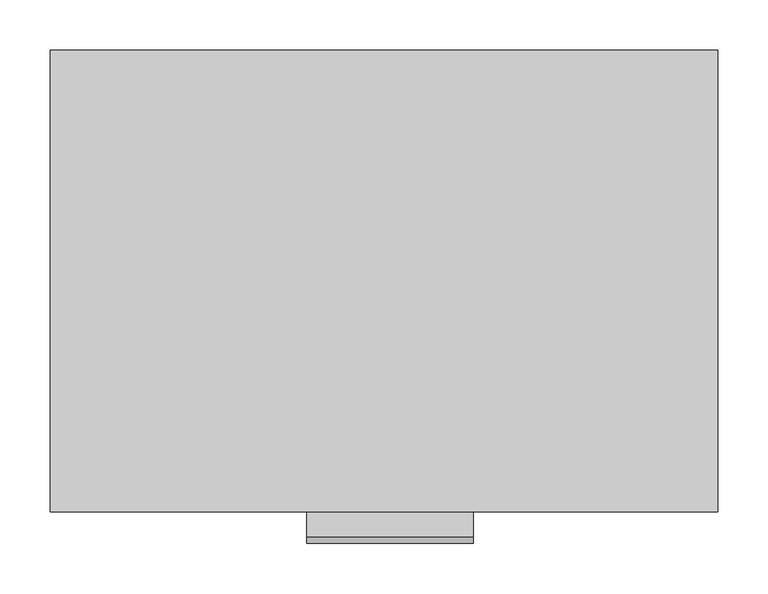
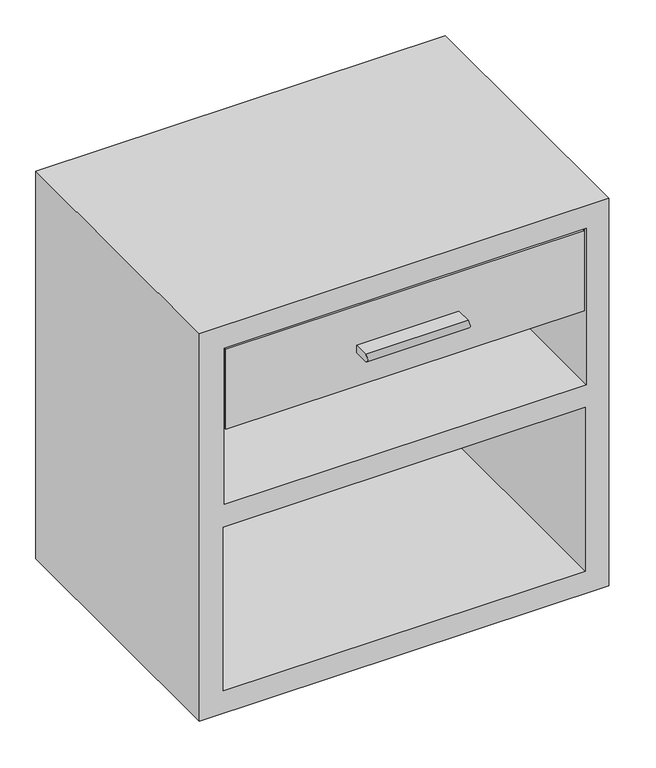
"""IFC4 building model written with IfcOpenShell, lengths in millimetres: furniture geometry, Livia_1_Drawer_Nightstand_20913 : Livia_1_Drawer_Nightstand_20913."""

import ifcopenshell
import ifcopenshell.guid

model = None  # the IFC model being written
_history = None  # IfcOwnerHistory: only IFC2X3 demands one
_inside = {}  # id of a spatial element -> (the spatial element, [elements in it])
_under = {}  # id of a project, library or spatial element -> (it, [spatial elements below it])
_declared = {}  # id of a project -> (the project, [libraries it declares])
_typed = {}  # id of a type object -> (the type object, [elements of that type])
_made_of = {}  # id of a material, layer set ... -> (it, [elements and type objects made of it])


def new_model(schema):
    """Start an empty IFC model of exactly this schema.

    Asked for "IFC4X3", IfcOpenShell would pick the latest addendum, in which some entities
    have other attributes; the version numbers below select the first issue.
    IFC2X3 requires an IfcOwnerHistory on every rooted entity: one is made here for all.
    """
    global model, _history
    if schema == "IFC4X3":
        model = ifcopenshell.file(schema_version=(4, 3, 0, 0))
    else:
        model = ifcopenshell.file(schema=schema)
    _inside.clear()
    _under.clear()
    _declared.clear()
    _typed.clear()
    _made_of.clear()
    _history = None
    if model.schema == "IFC2X3":
        org = make("IfcOrganization", Name="unknown")
        user = make(
            "IfcPersonAndOrganization",
            ThePerson=make("IfcPerson", FamilyName="unknown"),
            TheOrganization=org,
        )
        app = make(
            "IfcApplication",
            ApplicationDeveloper=org,
            Version="unknown",
            ApplicationFullName="unknown",
            ApplicationIdentifier="unknown",
        )
        _history = make(
            "IfcOwnerHistory",
            OwningUser=user,
            OwningApplication=app,
            ChangeAction="ADDED",
            CreationDate=0,
        )
    return model


def make(cls, **values):
    """One entity of the class cls with the attributes given. An attribute that is None is left unset."""
    return model.create_entity(
        cls, **{name: value for name, value in values.items() if value is not None}
    )


def rooted(cls, **values):
    """An entity with a GlobalId (a new one), such as an element, a storey or a relation."""
    return make(cls, GlobalId=ifcopenshell.guid.new(), OwnerHistory=_history, **values)


def si_unit(unit_type, name, prefix=None):
    """IfcSIUnit, for example si_unit("LENGTHUNIT", "METRE", prefix="MILLI")."""
    return make("IfcSIUnit", UnitType=unit_type, Prefix=prefix, Name=name)


def assignment(units):
    """IfcUnitAssignment: the units of a project."""
    return None if units is None else make("IfcUnitAssignment", Units=units)


def point(xyz):
    """IfcCartesianPoint."""
    return None if xyz is None else make("IfcCartesianPoint", Coordinates=xyz)


def direction(xyz):
    """IfcDirection."""
    return None if xyz is None else make("IfcDirection", DirectionRatios=xyz)


def frame(location, z_axis=None, x_axis=None):
    """IfcAxis2Placement3D, a coordinate frame: its origin and axes. An axis left out is left unset."""
    return make(
        "IfcAxis2Placement3D",
        Location=point(location),
        Axis=direction(z_axis),
        RefDirection=direction(x_axis),
    )


def origin():
    """The frame at (0, 0, 0) with its axes left unset."""
    return frame((0.0, 0.0, 0.0))


def place(relative_to, where):
    """IfcLocalPlacement: puts the frame where relative to a parent placement (None: the world)."""
    return make(
        "IfcLocalPlacement", PlacementRelTo=relative_to, RelativePlacement=where
    )


def context(
    kind, dimensions, precision=None, world=None, true_north=None, identifier=None
):
    """IfcGeometricRepresentationContext, for example the 3D "Model" context."""
    return make(
        "IfcGeometricRepresentationContext",
        ContextIdentifier=identifier,
        ContextType=kind,
        CoordinateSpaceDimension=dimensions,
        Precision=precision,
        WorldCoordinateSystem=world,
        TrueNorth=true_north,
    )


def project(units=None, contexts=None):
    """IfcProject with its units and contexts."""
    return rooted(
        "IfcProject",
        Name="project",
        RepresentationContexts=contexts,
        UnitsInContext=assignment(units),
    )


def spatial(cls, under=None, at=None, **own):
    """A site, building, storey or space (cls), placed at a placement, below another one or the project."""
    s = rooted(cls, ObjectPlacement=at, **own)
    if under is not None:
        _under.setdefault(under.id(), (under, []))[1].append(s)
    return s


def faces_of(points, faces, orient=None, outer=None):
    """IfcFace entities. A face is a list of loops; a loop is a list of indices into points, from 0.

    orient and outer hold one flag for each loop. By default every Orientation is true, the
    first loop of a face is its IfcFaceOuterBound and the others are IfcFaceBound.
    """
    made = []
    for i, loops in enumerate(faces):
        bounds = []
        for j, loop in enumerate(loops):
            is_outer = j == 0 if outer is None else outer[i][j]
            bounds.append(
                make(
                    "IfcFaceOuterBound" if is_outer else "IfcFaceBound",
                    Bound=make("IfcPolyLoop", Polygon=[points[k] for k in loop]),
                    Orientation=True if orient is None else orient[i][j],
                )
            )
        made.append(make("IfcFace", Bounds=bounds))
    return made


def faceted_brep(points, faces, orient=None, outer=None, voids=None):
    """IfcFacetedBrep: a solid bounded by flat faces; with voids (closed shells), ...WithVoids."""
    shared = [point(p) for p in points]
    hull = make("IfcClosedShell", CfsFaces=faces_of(shared, faces, orient, outer))
    if voids is None:
        return make("IfcFacetedBrep", Outer=hull)
    return make(
        "IfcFacetedBrepWithVoids",
        Outer=hull,
        Voids=[
            make(cls, CfsFaces=faces_of(shared, fs, o, b)) for cls, fs, o, b in voids
        ],
    )


def shape(context_of_items, identifier, shape_type, items):
    """IfcShapeRepresentation: the items that make up one representation, for example the "Body"."""
    return make(
        "IfcShapeRepresentation",
        ContextOfItems=context_of_items,
        RepresentationIdentifier=identifier,
        RepresentationType=shape_type,
        Items=items,
    )


def source(mapping_origin, context_of_items, identifier, shape_type, items):
    """IfcRepresentationMap: a shape defined once, which mapped items show again and again."""
    return make(
        "IfcRepresentationMap",
        MappingOrigin=mapping_origin,
        MappedRepresentation=shape(context_of_items, identifier, shape_type, items),
    )


def transform(
    local_origin,
    x_axis=None,
    y_axis=None,
    z_axis=None,
    scale=None,
    scale2=None,
    scale3=None,
    uniform=True,
):
    """IfcCartesianTransformationOperator3D, or its non-uniform kind. x_axis, y_axis, z_axis: its Axis1, 2, 3."""
    if uniform:
        return make(
            "IfcCartesianTransformationOperator3D",
            Axis1=direction(x_axis),
            Axis2=direction(y_axis),
            LocalOrigin=point(local_origin),
            Scale=scale,
            Axis3=direction(z_axis),
        )
    return make(
        "IfcCartesianTransformationOperator3DnonUniform",
        Axis1=direction(x_axis),
        Axis2=direction(y_axis),
        LocalOrigin=point(local_origin),
        Scale=scale,
        Axis3=direction(z_axis),
        Scale2=scale2,
        Scale3=scale3,
    )


def mapped(mapping_source, mapping_target):
    """IfcMappedItem: shows the shape of a source again, moved by a transform."""
    return make(
        "IfcMappedItem", MappingSource=mapping_source, MappingTarget=mapping_target
    )


def made_of(thing, what):
    """Note that an element or type object is made of a material, layer set ...; save() writes the relation."""
    if what is not None:
        _made_of.setdefault(what.id(), (what, []))[1].append(thing)
    return thing


def element(
    cls,
    number,
    at=None,
    inside=None,
    cuts=None,
    type_object=None,
    material=None,
    context=None,
    identifier="Body",
    shape_type=None,
    held_by="IfcProductDefinitionShape",
    body=None,
    shapes=None,
    **own,
):
    """One element of the class cls, such as IfcWall. Its Tag is "e" and its number.

    at: its placement. inside: the storey or other place that contains it. cuts: it is an
    opening in that element (IfcRelVoidsElement). A single representation is given by context,
    identifier, shape_type and body (its items); several are given by shapes. held_by: the class
    of the entity that holds the representations. save() writes the other relations.
    """
    e = rooted(cls, Tag="e%d" % number, ObjectPlacement=at, **own)
    if body is not None:
        shapes = [shape(context, identifier, shape_type, body)]
    if shapes is not None:
        e.Representation = make(held_by, Representations=shapes)
    if inside is not None:
        _inside.setdefault(inside.id(), (inside, []))[1].append(e)
    if cuts is not None:
        rooted(
            "IfcRelVoidsElement", RelatingBuildingElement=cuts, RelatedOpeningElement=e
        )
    if type_object is not None:
        _typed.setdefault(type_object.id(), (type_object, []))[1].append(e)
    return made_of(e, material)


def aggregate(whole, parts):
    """IfcRelAggregates: a whole, such as a stair, and the parts it consists of."""
    return rooted("IfcRelAggregates", RelatingObject=whole, RelatedObjects=parts)


def save(model, path):
    """Write the relations noted so far, then the file.

    IfcRelAggregates (storeys below a building ...), IfcRelContainedInSpatialStructure (elements
    in a storey), IfcRelDefinesByType, IfcRelAssociatesMaterial and IfcRelDeclares: one each for
    every whole, place, type object, material and project.
    """
    for whole, parts in _under.values():
        aggregate(whole, parts)
    for where, things in _inside.values():
        rooted(
            "IfcRelContainedInSpatialStructure",
            RelatedElements=things,
            RelatingStructure=where,
        )
    for kind, things in _typed.values():
        rooted("IfcRelDefinesByType", RelatedObjects=things, RelatingType=kind)
    for what, things in _made_of.values():
        rooted("IfcRelAssociatesMaterial", RelatedObjects=things, RelatingMaterial=what)
    for by, libraries in _declared.values():
        rooted("IfcRelDeclares", RelatingContext=by, RelatedDefinitions=libraries)
    model.write(path)


def plane_surface(at):
    """IfcPlane: the flat surface through the origin of the frame at, square to its z axis."""
    return make("IfcPlane", Position=at)


def extruded_surface(curve, direction_of_extrusion, depth):
    """IfcSurfaceOfLinearExtrusion: the curve pushed along a direction by depth."""
    return make(
        "IfcSurfaceOfLinearExtrusion",
        SweptCurve=make("IfcArbitraryOpenProfileDef", ProfileType="CURVE", Curve=curve),
        ExtrudedDirection=direction(direction_of_extrusion),
        Depth=depth,
    )


def spline_curve(degree, points, multiplicities, knots, weights=None):
    """IfcBSplineCurveWithKnots; with weights, IfcRationalBSplineCurveWithKnots."""
    own = dict(
        Degree=degree,
        ControlPointsList=[point(p) for p in points],
        CurveForm="UNSPECIFIED",
        ClosedCurve=False,
        SelfIntersect=False,
        KnotMultiplicities=multiplicities,
        Knots=knots,
        KnotSpec="UNSPECIFIED",
    )
    if weights is None:
        return make("IfcBSplineCurveWithKnots", **own)
    return make("IfcRationalBSplineCurveWithKnots", WeightsData=weights, **own)


def advanced_brep(points, edges, surfaces, faces):
    """IfcAdvancedBrep: a solid bounded by faces that lie on surfaces and meet in shared edges.

    An edge is (start, end): straight between two places in points (the first is 0);
    or (start, end, curve); or (start, end, curve, False) where it runs against its curve.
    A face is (place in surfaces, loops), or (place, loops, False) where it looks against
    its surface's normal. A loop lists edges by number (the first is 1), with a minus sign
    where the edge is run from its end to its start. The first loop is the outer one.
    """
    corners = [point(p) for p in points]
    vertices = [make("IfcVertexPoint", VertexGeometry=c) for c in corners]
    made = []
    for start, end, *more in edges:
        made.append(
            make(
                "IfcEdgeCurve",
                EdgeStart=vertices[start],
                EdgeEnd=vertices[end],
                EdgeGeometry=more[0] if more else make("IfcPolyline", Points=[corners[start], corners[end]]),
                SameSense=more[1] if len(more) > 1 else True,
            )
        )
    hull = []
    for where, loops, *sense in faces:
        bounds = []
        for j, loop in enumerate(loops):
            ring = [make("IfcOrientedEdge", EdgeElement=made[abs(k) - 1], Orientation=k > 0) for k in loop]
            bounds.append(
                make(
                    "IfcFaceOuterBound" if j == 0 else "IfcFaceBound",
                    Bound=make("IfcEdgeLoop", EdgeList=ring),
                    Orientation=True,
                )
            )
        hull.append(make("IfcAdvancedFace", Bounds=bounds, FaceSurface=surfaces[where], SameSense=sense[0] if sense else True))
    return make("IfcAdvancedBrep", Outer=make("IfcClosedShell", CfsFaces=hull))


def furniture_23f017af(model_context):
    return source(origin(), model_context, "Body", "SolidModel", [
        advanced_brep(
        [(-76.575761, -228.6, 552.45), (-76.575761, -228.6, 539.75), (-76.575761, -254.0, 539.75), (-76.575761, -254.0, 552.45), (88.524239, -228.6, 552.45), (88.524239, -254.0, 552.45), (88.524239, -254.0, 539.75), (88.524239, -228.6, 539.75)],
        [
            (0, 1),
            (1, 2),
            (2, 3, spline_curve(3, [(-76.575761, -254.0, 539.75), (-76.575761, -261.758833332, 543.737102154), (-76.575761, -261.758833332, 547.970435488), (-76.575761, -254.0, 552.45)], [4, 4], [0.0, 0.04350998662349671])),
            (3, 0),
            (4, 5),
            (5, 6, spline_curve(3, [(88.524239, -254.0, 552.45), (88.524239, -261.758833332, 547.970435488), (88.524239, -261.758833332, 543.737102154), (88.524239, -254.0, 539.75)], [4, 4], [0.0, 0.04350998662349671])),
            (6, 7),
            (7, 4),
            (0, 4),
            (7, 1),
            (6, 2),
            (5, 3),
        ],
        [
            plane_surface(frame((-76.575761, -228.6, 545.7306532), z_axis=(-1.0, 0.0, 0.0), x_axis=(0.0, -1.0, 0.0))),
            plane_surface(frame((88.524239, -228.6, 545.7306532), z_axis=(1.0, 0.0, 0.0), x_axis=(0.0, -1.0, 0.0))),
            plane_surface(frame((-76.575761, -228.6, 552.45), z_axis=(0.0, 1.0, 0.0), x_axis=(1.0, 0.0, 0.0))),
            plane_surface(frame((-76.575761, -228.6, 539.75), z_axis=(0.0, 0.0, -1.0), x_axis=(1.0, 0.0, 0.0))),
            extruded_surface(spline_curve(3, [(88.524239, -254.0, 539.75), (88.524239, -261.758833332, 543.737102154), (88.524239, -261.758833332, 547.970435488), (88.524239, -254.0, 552.45)], [4, 4], [0.0, 0.04350998662349671]), (-165.1, 0.0, 0.0), 165.1),
            plane_surface(frame((-76.575761, -254.0, 552.45), z_axis=(0.0, 0.0, 1.0), x_axis=(1.0, 0.0, 0.0))),
        ],
        [
            (0, [[1, 2, 3, 4]]),
            (1, [[5, 6, 7, 8]]),
            (2, [[-1, 9, -8, 10]]),
            (3, [[-2, -10, -7, 11]]),
            (4, [[-3, -11, -6, 12]]),
            (5, [[-4, -12, -5, -9]]),
        ],
    ),
        faceted_brep([(330.2, -228.6, 0.0), (330.2, -228.6, 660.4), (-330.2, -228.6, 660.4), (-330.2, -228.6, 0.0), (292.1, -228.6, 317.5), (292.1, -228.6, 38.1), (-292.1, -228.6, 38.1), (-292.1, -228.6, 317.5), (293.7115278, -228.6, 622.3), (293.7115278, -228.6, 355.6), (-290.4884722, -228.6, 355.6), (-290.4884722, -228.6, 622.3), (-287.3134722, -228.6, 482.6), (290.5365278, -228.6, 482.6), (290.5365278, -228.6, 619.125), (-287.3134722, -228.6, 619.125), (330.2, 228.6, 0.0), (-330.2, 228.6, 0.0), (-330.2, 228.6, 660.4), (330.2, 228.6, 660.4), (292.1, 228.6, 38.1), (292.1, 228.6, 317.5), (-292.1, 228.6, 317.5), (-292.1, 228.6, 38.1), (293.7115278, 228.6, 355.6), (293.7115278, 228.6, 482.6), (-290.4884722, 228.6, 482.6), (-290.4884722, 228.6, 355.6), (293.7115278, -223.8644244, 622.3), (293.7115278, -223.8644244, 482.6), (290.5365278, -223.8644244, 482.6), (-287.3134722, -223.8644244, 482.6), (-290.4884722, -223.8644244, 482.6), (-290.4884722, -223.8644244, 622.3), (-287.3134722, -223.8644244, 619.125), (290.5365278, -223.8644244, 619.125)], [[[0, 1, 2, 3], [4, 5, 6, 7], [8, 9, 10, 11]], [[12, 13, 14, 15]], [[16, 17, 18, 19], [20, 21, 22, 23], [24, 25, 26, 27]], [[1, 0, 16, 19]], [[2, 1, 19, 18]], [[3, 2, 18, 17]], [[0, 3, 17, 16]], [[20, 5, 4, 21]], [[21, 4, 7, 22]], [[22, 7, 6, 23]], [[5, 20, 23, 6]], [[24, 9, 8, 28, 29, 25]], [[26, 25, 29, 30, 13, 12, 31, 32]], [[10, 27, 26, 32, 33, 11]], [[9, 24, 27, 10]], [[33, 32, 31, 34, 35, 30, 29, 28]], [[34, 31, 12, 15]], [[35, 34, 15, 14]], [[30, 35, 14, 13]], [[33, 28, 8, 11]]]),
    ])


if __name__ == "__main__":
    model = new_model("IFC4")
    model_context = context("Model", 3, world=origin())
    ifc_project = project(units=[si_unit("LENGTHUNIT", "METRE", prefix="MILLI")], contexts=[model_context])
    site = spatial("IfcSite", under=ifc_project)
    building = spatial("IfcBuilding", under=site)
    placement = place(None, origin())
    furniture_shape = furniture_23f017af(model_context)
    element("IfcFurniture", 1, ObjectType="Livia_1_Drawer_Nightstand_20913 : Livia_1_Drawer_Nightstand_20913", at=placement, inside=building, context=model_context, shape_type="MappedRepresentation", body=[
        mapped(furniture_shape, transform((0.0, 0.0, 0.0), x_axis=(1.0, 0.0, 0.0), y_axis=(0.0, 1.0, 0.0), z_axis=(0.0, 0.0, 1.0))),
    ])
    save(model, "model.ifc")

# Revit data of these elements
# Type "Livia_1_Drawer_Nightstand_20913 : Livia_1_Drawer_Nightstand_20913"
#   Width = 0.6604 m
#   Depth = 0.4572 m
#   Side Table Material = none
#   Drawer Pull = none
#   Default Elevation = 0
